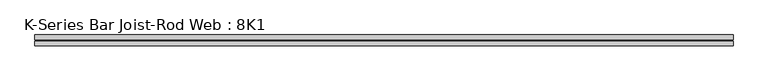
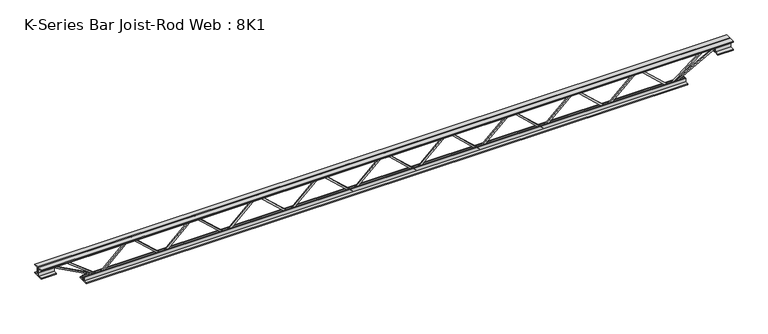
"""IFC4 building model written with IfcOpenShell, lengths in millimetres: beam geometry, K-Series Bar Joist-Rod Web : 8K1."""

from ifc_helpers import new_model, si_unit, frame, origin, place, context, project, spatial, polyline, outline, extrude, source, transform, mapped, element, save


def k_series_bar_joist_rod_web_8k1_1f0329fa(model_context):
    return source(origin(), model_context, "Body", "SweptSolid", [
        extrude(outline(polyline([(-90.4875, 1067.8380982), (-100.0125, 1067.8380982), (-100.0125, 1072.8695868), (90.4875, 1280.0872064), (90.4875, 1282.7242294), (-100.0125, 1489.941849), (-100.0125, 1494.9733375), (-90.4875, 1494.9733375), (-90.4875, 1493.654826), (100.0125, 1286.4372064), (100.0125, 1276.3742294), (-90.4875, 1069.1566097), (-90.4875, 1067.8380982)])), frame((0.0, -4.7625, 0.0), z_axis=(0.0, 1.0, 0.0), x_axis=(0.0, 0.0, 1.0)), (0.0, 0.0, 1.0), 9.525),
        extrude(outline(polyline([(-90.4875, 640.7028589), (-100.0125, 640.7028589), (-100.0125, 645.7343475), (90.4875, 852.9519671), (90.4875, 855.5889901), (-100.0125, 1062.8066097), (-100.0125, 1067.8380982), (-90.4875, 1067.8380982), (-90.4875, 1066.5195868), (100.0125, 859.3019671), (100.0125, 849.2389901), (-90.4875, 642.0213704), (-90.4875, 640.7028589)])), frame((0.0, -4.7625, 0.0), z_axis=(0.0, 1.0, 0.0), x_axis=(0.0, 0.0, 1.0)), (0.0, 0.0, 1.0), 9.525),
        extrude(outline(polyline([(-90.4875, 213.5676196), (-100.0125, 213.5676196), (-100.0125, 218.5991082), (90.4875, 425.8167278), (90.4875, 428.4537508), (-100.0125, 635.6713704), (-100.0125, 640.7028589), (-90.4875, 640.7028589), (-90.4875, 639.3843475), (100.0125, 432.1667278), (100.0125, 422.1037508), (-90.4875, 214.8861311), (-90.4875, 213.5676196)])), frame((0.0, -4.7625, 0.0), z_axis=(0.0, 1.0, 0.0), x_axis=(0.0, 0.0, 1.0)), (0.0, 0.0, 1.0), 9.525),
        extrude(outline(polyline([(-90.4875, -213.5676196), (-100.0125, -213.5676196), (-100.0125, -208.5361311), (90.4875, -1.3185115), (90.4875, 1.3185115), (-100.0125, 208.5361311), (-100.0125, 213.5676196), (-90.4875, 213.5676196), (-90.4875, 212.2491082), (100.0125, 5.0314885), (100.0125, -5.0314885), (-90.4875, -212.2491082), (-90.4875, -213.5676196)])), frame((0.0, -4.7625, 0.0), z_axis=(0.0, 1.0, 0.0), x_axis=(0.0, 0.0, 1.0)), (0.0, 0.0, 1.0), 9.525),
        extrude(outline(polyline([(-90.4875, -640.7028589), (-100.0125, -640.7028589), (-100.0125, -635.6713704), (90.4875, -428.4537508), (90.4875, -425.8167278), (-100.0125, -218.5991082), (-100.0125, -213.5676196), (-90.4875, -213.5676196), (-90.4875, -214.8861311), (100.0125, -422.1037508), (100.0125, -432.1667278), (-90.4875, -639.3843475), (-90.4875, -640.7028589)])), frame((0.0, -4.7625, 0.0), z_axis=(0.0, 1.0, 0.0), x_axis=(0.0, 0.0, 1.0)), (0.0, 0.0, 1.0), 9.525),
        extrude(outline(polyline([(-90.4875, -1067.8380982), (-100.0125, -1067.8380982), (-100.0125, -1062.8066097), (90.4875, -855.5889901), (90.4875, -852.9519671), (-100.0125, -645.7343475), (-100.0125, -640.7028589), (-90.4875, -640.7028589), (-90.4875, -642.0213704), (100.0125, -849.2389901), (100.0125, -859.3019671), (-90.4875, -1066.5195868), (-90.4875, -1067.8380982)])), frame((0.0, -4.7625, 0.0), z_axis=(0.0, 1.0, 0.0), x_axis=(0.0, 0.0, 1.0)), (0.0, 0.0, 1.0), 9.525),
        extrude(outline(polyline([(-90.4875, -1494.9733375), (-100.0125, -1494.9733375), (-100.0125, -1489.941849), (90.4875, -1282.7242294), (90.4875, -1280.0872064), (-100.0125, -1072.8695868), (-100.0125, -1067.8380982), (-90.4875, -1067.8380982), (-90.4875, -1069.1566097), (100.0125, -1276.3742294), (100.0125, -1286.4372064), (-90.4875, -1493.654826), (-90.4875, -1494.9733375)])), frame((0.0, -4.7625, 0.0), z_axis=(0.0, 1.0, 0.0), x_axis=(0.0, 0.0, 1.0)), (0.0, 0.0, 1.0), 9.525),
        extrude(outline(polyline([(-90.4875, 1494.9733375), (-100.0125, 1494.9733375), (-100.0125, 1500.004826), (90.4875, 1707.2224457), (90.4875, 1709.8594686), (-100.0125, 1917.0770883), (-100.0125, 1922.1085768), (-90.4875, 1922.1085768), (-90.4875, 1920.7900653), (100.0125, 1713.5724457), (100.0125, 1703.5094686), (-90.4875, 1496.291849), (-90.4875, 1494.9733375)])), frame((0.0, -4.7625, 0.0), z_axis=(0.0, 1.0, 0.0), x_axis=(0.0, 0.0, 1.0)), (0.0, 0.0, 1.0), 9.525),
        extrude(outline(polyline([(-90.4875, -1922.1085768), (-100.0125, -1922.1085768), (-100.0125, -1917.0770883), (90.4875, -1709.8594686), (90.4875, -1707.2224457), (-100.0125, -1500.004826), (-100.0125, -1494.9733375), (-90.4875, -1494.9733375), (-90.4875, -1496.291849), (100.0125, -1703.5094686), (100.0125, -1713.5724457), (-90.4875, -1920.7900653), (-90.4875, -1922.1085768)])), frame((0.0, -4.7625, 0.0), z_axis=(0.0, 1.0, 0.0), x_axis=(0.0, 0.0, 1.0)), (0.0, 0.0, 1.0), 9.525),
        extrude(outline(polyline([(4.7625, 101.6), (36.5125, 101.6), (36.5125, 95.25), (11.1125, 95.25), (11.1125, 69.85), (4.7625, 69.85), (4.7625, 101.6)])), frame((-2328.5085768, 0.0, 0.0), z_axis=(1.0, 0.0, 0.0), x_axis=(0.0, 1.0, 0.0)), (0.0, 0.0, 1.0), 4657.0171536),
        extrude(outline(polyline([(-4.7625, 101.6), (-4.7625, 69.85), (-11.1125, 69.85), (-11.1125, 95.25), (-36.5125, 95.25), (-36.5125, 101.6), (-4.7625, 101.6)])), frame((-2328.5085768, 0.0, 0.0), z_axis=(1.0, 0.0, 0.0), x_axis=(0.0, 1.0, 0.0)), (0.0, 0.0, 1.0), 4657.0171536),
        extrude(outline(polyline([(-4.7625, 38.1), (-36.5125, 38.1), (-36.5125, 44.45), (-11.1125, 44.45), (-11.1125, 69.85), (-4.7625, 69.85), (-4.7625, 38.1)])), frame((-2328.5085768, 0.0, 0.0), z_axis=(1.0, 0.0, 0.0), x_axis=(0.0, 1.0, 0.0)), (0.0, 0.0, 1.0), 101.6),
        extrude(outline(polyline([(36.5125, 38.1), (4.7625, 38.1), (4.7625, 69.85), (11.1125, 69.85), (11.1125, 44.45), (36.5125, 44.45), (36.5125, 38.1)])), frame((-2328.5085768, 0.0, 0.0), z_axis=(1.0, 0.0, 0.0), x_axis=(0.0, 1.0, 0.0)), (0.0, 0.0, 1.0), 101.6),
        extrude(outline(polyline([(4.7625, 38.1), (4.7625, 69.85), (11.1125, 69.85), (11.1125, 44.45), (36.5125, 44.45), (36.5125, 38.1), (4.7625, 38.1)])), frame((2226.9085768, 0.0, 0.0), z_axis=(1.0, 0.0, 0.0), x_axis=(0.0, 1.0, 0.0)), (0.0, 0.0, 1.0), 101.6),
        extrude(outline(polyline([(-4.7625, 38.1), (-36.5125, 38.1), (-36.5125, 44.45), (-11.1125, 44.45), (-11.1125, 69.85), (-4.7625, 69.85), (-4.7625, 38.1)])), frame((2226.9085768, 0.0, 0.0), z_axis=(1.0, 0.0, 0.0), x_axis=(0.0, 1.0, 0.0)), (0.0, 0.0, 1.0), 101.6),
        extrude(outline(polyline([(4.7625, -101.6), (4.7625, -69.85), (11.1125, -69.85), (11.1125, -95.25), (36.5125, -95.25), (36.5125, -101.6), (4.7625, -101.6)])), frame((-2023.7085768, 0.0, 0.0), z_axis=(1.0, 0.0, 0.0), x_axis=(0.0, 1.0, 0.0)), (0.0, 0.0, 1.0), 4047.4171536),
        extrude(outline(polyline([(-4.7625, -101.6), (-36.5125, -101.6), (-36.5125, -95.25), (-11.1125, -95.25), (-11.1125, -69.85), (-4.7625, -69.85), (-4.7625, -101.6)])), frame((-2023.7085768, 0.0, 0.0), z_axis=(1.0, 0.0, 0.0), x_axis=(0.0, 1.0, 0.0)), (0.0, 0.0, 1.0), 4047.4171536),
        extrude(outline(polyline([(0.0, -9.525), (0.0, 0.0), (346.6425392, 0.0), (346.6425392, -9.525), (0.0, -9.525)])), frame((-2229.1768753, 4.7625, 65.662372), z_axis=(0.47628314854008075, 0.0, 0.879291966537138), x_axis=(0.879291966537138, 0.0, -0.47628314854008075)), (0.0, 0.0, 1.0), 9.525),
        extrude(outline(polyline([(0.0, -9.525), (0.0, 0.0), (269.9428424, 0.0), (269.9428424, -9.525), (0.0, -9.525)])), frame((-2138.5889936, 4.7625, 66.0821068), z_axis=(0.6116109563555343, 0.0, 0.7911586680722577), x_axis=(0.7911586680722577, 0.0, -0.6116109563555343)), (0.0, 0.0, 1.0), 9.525),
        extrude(outline(polyline([(0.0, -9.525), (0.0, 0.0), (346.6425392, 0.0), (346.6425392, -9.525), (0.0, -9.525)])), frame((2229.1768753, -4.7625, 65.662372), z_axis=(-0.4762831485400419, 0.0, 0.8792919665371591), x_axis=(-0.8792919665371591, 0.0, -0.4762831485400419)), (0.0, 0.0, 1.0), 9.525),
        extrude(outline(polyline([(0.0, -9.525), (0.0, 0.0), (269.9428424, 0.0), (269.9428424, -9.525), (0.0, -9.525)])), frame((2138.5889936, -4.7625, 66.0821068), z_axis=(-0.6116109563555123, 0.0, 0.7911586680722746), x_axis=(-0.7911586680722746, 0.0, -0.6116109563555123)), (0.0, 0.0, 1.0), 9.525),
    ])


if __name__ == "__main__":
    model = new_model("IFC4")
    model_context = context("Model", 3, world=origin())
    ifc_project = project(units=[si_unit("LENGTHUNIT", "METRE", prefix="MILLI")], contexts=[model_context])
    site = spatial("IfcSite", under=ifc_project)
    building = spatial("IfcBuilding", under=site)
    placement = place(None, origin())
    k_series_bar_joist_rod_web_8k1_shape = k_series_bar_joist_rod_web_8k1_1f0329fa(model_context)
    element("IfcBeam", 1, ObjectType="K-Series Bar Joist-Rod Web : 8K1", at=placement, inside=building, context=model_context, shape_type="MappedRepresentation", body=[
        mapped(k_series_bar_joist_rod_web_8k1_shape, transform((0.0, 0.0, 0.0), x_axis=(1.0, 0.0, 0.0), y_axis=(0.0, 1.0, 0.0), z_axis=(0.0, 0.0, 1.0))),
    ])
    save(model, "model.ifc")

# Revit data of these elements
# Type "K-Series Bar Joist-Rod Web : 8K1"
#   Assembly Code = "B1010350"
#   Wt = 5.1
#   Web Thickness = 0' - 0 3/8"
#   Start Offset [instance default] = 0' - 0"
#   Start Extension [instance default] = 0' - 0"
#   Seat Length = 0' - 4"
#   Seat Depth = 0' - 2 1/2"
#   PanelArrayLength [instance default] = 21' - 4"
#   Panel [instance default] = 1' - 4"
#   End Offset [instance default] = 0' - 0"
#   End Extension [instance default] = 0' - 0"
#   End Panel = 1' - 4"
#   Cord Leg = 0' - 1 1/4"
#   Chord Thickness = 0' - 0 1/4"
#   Length [instance default] = 24' - 0"
#   Depth = 0' - 8"
#   PanelArrayNum [instance default] = 16
#   Rendering Material = none
# Element 1 (IfcBeam, "K-Series Bar Joist-Rod Web : 8K1")
#   PanelArrayLength = 12' - 7.34713"
#   Panel = 1' - 4.81635"
#   PanelArrayNum = 9
